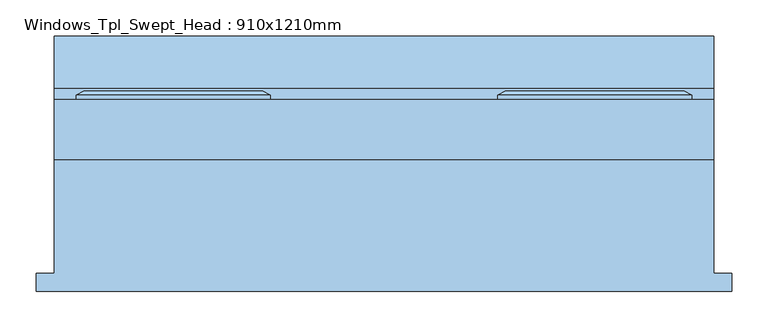
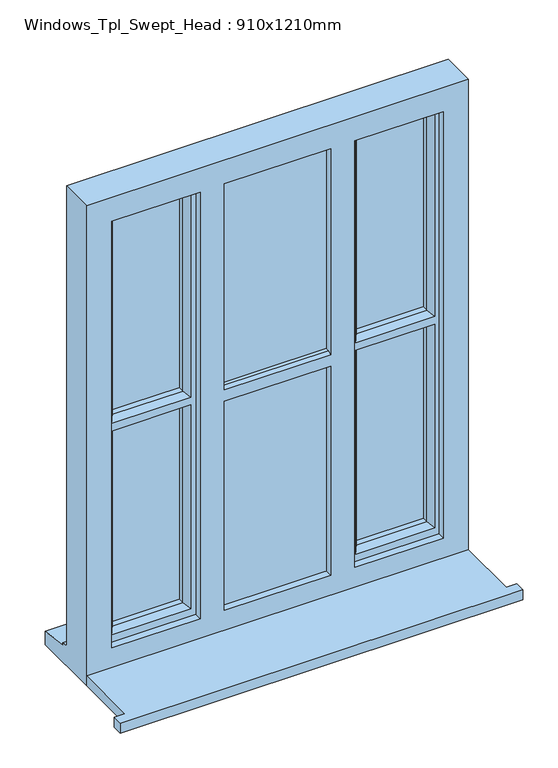
"""IFC4 building model written with IfcOpenShell, lengths in millimetres: window geometry, Windows_Tpl_Swept_Head : 910x1210mm."""

from ifc_helpers import new_model, si_unit, point, frame, frame_2d, origin, place, context, project, spatial, polyline, circle_curve, trimmed, segment, composite_curve, outline, extrude, faceted_brep, source, transform, mapped, element, save


def windows_tpl_swept_head_910x1210mm_1738034d(model_context):
    return source(origin(), model_context, "Body", "SolidModel", [
        extrude(outline(polyline([(-906.6666667, -161.5434322), (-906.6666667, -136.5434322), (-881.6666667, -136.5434322), (-881.6666667, 20.4565678), (28.3333333, 20.4565678), (28.3333333, -136.5434322), (53.3333333, -136.5434322), (53.3333333, -161.5434322), (-906.6666667, -161.5434322)])), frame((0.0, 0.0, 900.0), z_axis=(0.0, 0.0, 1.0), x_axis=(1.0, 0.0, 0.0)), (0.0, 0.0, 1.0), 25.0),
        extrude(outline(composite_curve([segment(polyline([(2050.0, -300.0), (2050.0, -553.3333333), (2013.444301, -553.3333333)]), True, "CONTINUOUS"), segment(trimmed(circle_curve(frame_2d((1325.0, -426.6666667)), 700.0), [point((2013.444301, -553.3333333))], [point((2013.444301, -300.0))], True, "CARTESIAN"), True, "CONTINUOUS"), segment(polyline([(2013.444301, -300.0), (2050.0, -300.0)]), True, "CONTINUOUS")], self_intersect=False)), frame((0.0, 62.4565678, 0.0), z_axis=(0.0, 1.0, 0.0), x_axis=(0.0, 0.0, 1.0)), (0.0, 0.0, 1.0), 25.0),
        extrude(outline(composite_curve([segment(polyline([(2030.0, -220.0), (2019.9215583, -220.0)]), True, "CONTINUOUS"), segment(trimmed(circle_curve(frame_2d((1325.0, -135.8333333)), 700.0), [point((2019.9215583, -220.0))], [point((2019.9215583, -51.6666667))], True, "CARTESIAN"), True, "CONTINUOUS"), segment(polyline([(2019.9215583, -51.6666667), (2030.0, -51.6666667), (2030.0, -220.0)]), True, "CONTINUOUS")], self_intersect=False)), frame((0.0, 79.4565678, 0.0), z_axis=(0.0, 1.0, 0.0), x_axis=(0.0, 0.0, 1.0)), (0.0, 0.0, 1.0), 24.0),
        extrude(outline(composite_curve([segment(polyline([(2030.0, -633.3333333), (2030.0, -801.6666667), (2019.9215583, -801.6666667)]), True, "CONTINUOUS"), segment(trimmed(circle_curve(frame_2d((1325.0, -717.5)), 700.0), [point((2019.9215583, -801.6666667))], [point((2019.9215583, -633.3333333))], True, "CARTESIAN"), True, "CONTINUOUS"), segment(polyline([(2019.9215583, -633.3333333), (2030.0, -633.3333333)]), True, "CONTINUOUS")], self_intersect=False)), frame((0.0, 79.4565678, 0.0), z_axis=(0.0, 1.0, 0.0), x_axis=(0.0, 0.0, 1.0)), (0.0, 0.0, 1.0), 24.0),
        faceted_brep([(-270.0, 103.4565678, 2080.0), (-270.0, 109.2300705, 2080.0), (-270.0, 109.2300705, 953.0), (-270.0, 103.4565678, 953.0), (-260.0, 38.4565678, 2070.0), (-260.0, 103.4565678, 2070.0), (-260.0, 103.4565678, 963.0), (-260.0, 38.4565678, 963.0), (-220.0, 52.9494677, 2030.0), (-230.1480377, 38.4565678, 2040.1480377), (-230.1480377, 38.4565678, 1526.3519623), (-220.0, 52.9494677, 1536.5), (-230.1480377, 38.4565678, 992.8519623), (-220.0, 52.9494677, 1003.0), (-220.0, 52.9494677, 1496.5), (-230.1480377, 38.4565678, 1506.6480377), (-220.0, 67.4565678, 2030.0), (-220.0, 67.4565678, 1536.5), (-220.0, 67.4565678, 1003.0), (-220.0, 67.4565678, 1496.5), (-230.0, 91.4565678, 1529.5), (-230.0, 91.4565678, 2040.0), (-230.0, 67.4565678, 2040.0), (-230.0, 67.4565678, 1529.5), (-230.0, 67.4565678, 1503.5), (-230.0, 67.4565678, 993.0), (-230.0, 91.4565678, 993.0), (-230.0, 91.4565678, 1503.5), (-220.0, 109.2300705, 2030.0), (-220.0, 91.4565678, 2030.0), (-220.0, 91.4565678, 1536.5), (-220.0, 109.2300705, 1536.5), (-220.0, 91.4565678, 1003.0), (-220.0, 109.2300705, 1003.0), (-220.0, 109.2300705, 1496.5), (-220.0, 91.4565678, 1496.5), (-237.4457548, 115.0035732, 2047.4457548), (-237.4457548, 115.0035732, 1519.0542452), (-237.4457548, 115.0035732, 985.5542452), (-237.4457548, 115.0035732, 1513.9457548), (-259.2153903, 115.0035732, 2069.2153903), (-259.2153903, 115.0035732, 963.7846097), (-1.6666667, 109.2300705, 953.0), (-1.6666667, 103.4565678, 953.0), (-11.6666667, 103.4565678, 963.0), (-11.6666667, 38.4565678, 963.0), (-41.5186289, 38.4565678, 992.8519623), (-51.6666667, 52.9494677, 1003.0), (-51.6666667, 67.4565678, 1003.0), (-41.6666667, 67.4565678, 993.0), (-41.6666667, 91.4565678, 993.0), (-51.6666667, 91.4565678, 1003.0), (-51.6666667, 109.2300705, 1003.0), (-34.2209119, 115.0035732, 985.5542452), (-12.4512764, 115.0035732, 963.7846097), (-1.6666667, 109.2300705, 2080.0), (-1.6666667, 103.4565678, 2080.0), (-11.6666667, 103.4565678, 2070.0), (-11.6666667, 38.4565678, 2070.0), (-41.5186289, 38.4565678, 1506.6480377), (-51.6666667, 52.9494677, 1496.5), (-41.5186289, 38.4565678, 2040.1480377), (-51.6666667, 52.9494677, 2030.0), (-51.6666667, 52.9494677, 1536.5), (-41.5186289, 38.4565678, 1526.3519623), (-51.6666667, 67.4565678, 1496.5), (-51.6666667, 67.4565678, 2030.0), (-51.6666667, 67.4565678, 1536.5), (-41.6666667, 91.4565678, 1503.5), (-41.6666667, 67.4565678, 1503.5), (-41.6666667, 67.4565678, 1529.5), (-41.6666667, 67.4565678, 2040.0), (-41.6666667, 91.4565678, 2040.0), (-41.6666667, 91.4565678, 1529.5), (-51.6666667, 91.4565678, 1496.5), (-51.6666667, 109.2300705, 1496.5), (-51.6666667, 91.4565678, 2030.0), (-51.6666667, 109.2300705, 2030.0), (-51.6666667, 109.2300705, 1536.5), (-51.6666667, 91.4565678, 1536.5), (-34.2209119, 115.0035732, 1513.9457548), (-34.2209119, 115.0035732, 2047.4457548), (-34.2209119, 115.0035732, 1519.0542452), (-12.4512764, 115.0035732, 2069.2153903)], [[[0, 1, 2, 3]], [[4, 5, 6, 7]], [[8, 9, 10, 11]], [[12, 13, 14, 15]], [[16, 8, 11, 17]], [[13, 18, 19, 14]], [[20, 21, 22, 23]], [[24, 25, 26, 27]], [[28, 29, 30, 31]], [[32, 33, 34, 35]], [[36, 28, 31, 37]], [[33, 38, 39, 34]], [[2, 1, 40, 41]], [[3, 2, 42, 43]], [[7, 6, 44, 45]], [[13, 12, 46, 47]], [[18, 13, 47, 48]], [[26, 25, 49, 50]], [[33, 32, 51, 52]], [[38, 33, 52, 53]], [[2, 41, 54, 42]], [[43, 42, 55, 56]], [[45, 44, 57, 58]], [[47, 46, 59, 60]], [[61, 62, 63, 64]], [[48, 47, 60, 65]], [[62, 66, 67, 63]], [[68, 50, 49, 69]], [[70, 71, 72, 73]], [[52, 51, 74, 75]], [[76, 77, 78, 79]], [[53, 52, 75, 80]], [[77, 81, 82, 78]], [[42, 54, 83, 55]], [[1, 0, 56, 55]], [[0, 3, 43, 56], [6, 5, 57, 44]], [[5, 4, 58, 57]], [[4, 7, 45, 58], [46, 12, 15, 59], [61, 64, 10, 9]], [[9, 8, 62, 61]], [[8, 16, 66, 62]], [[49, 25, 24, 69], [18, 48, 65, 19]], [[22, 71, 70, 23], [66, 16, 17, 67]], [[22, 21, 72, 71]], [[26, 50, 68, 27], [32, 35, 74, 51]], [[72, 21, 20, 73], [76, 79, 30, 29]], [[29, 28, 77, 76]], [[28, 36, 81, 77]], [[41, 40, 83, 54], [36, 37, 82, 81], [38, 53, 80, 39]], [[40, 1, 55, 83]], [[82, 37, 31, 78]], [[30, 79, 78, 31]], [[73, 20, 23, 70]], [[11, 63, 67, 17]], [[10, 64, 63, 11]], [[59, 15, 14, 60]], [[60, 14, 19, 65]], [[27, 68, 69, 24]], [[74, 35, 34, 75]], [[39, 80, 75, 34]]]),
        faceted_brep([(-583.3333333, 103.4565678, 2080.0), (-583.3333333, 109.2300705, 2080.0), (-851.6666667, 109.2300705, 2080.0), (-851.6666667, 103.4565678, 2080.0), (-593.3333333, 38.4565678, 2070.0), (-593.3333333, 103.4565678, 2070.0), (-841.6666667, 103.4565678, 2070.0), (-841.6666667, 38.4565678, 2070.0), (-633.3333333, 52.9494677, 2030.0), (-623.1852956, 38.4565678, 2040.1480377), (-811.8147044, 38.4565678, 2040.1480377), (-801.6666667, 52.9494677, 2030.0), (-801.6666667, 67.4565678, 2030.0), (-633.3333333, 67.4565678, 2030.0), (-623.3333333, 91.4565678, 2040.0), (-623.3333333, 67.4565678, 2040.0), (-811.6666667, 67.4565678, 2040.0), (-811.6666667, 91.4565678, 2040.0), (-633.3333333, 109.2300705, 2030.0), (-633.3333333, 91.4565678, 2030.0), (-801.6666667, 91.4565678, 2030.0), (-801.6666667, 109.2300705, 2030.0), (-819.1124215, 115.0035732, 2047.4457548), (-615.8875785, 115.0035732, 2047.4457548), (-594.117943, 115.0035732, 2069.2153903), (-840.882057, 115.0035732, 2069.2153903), (-851.6666667, 109.2300705, 953.0), (-851.6666667, 103.4565678, 953.0), (-841.6666667, 103.4565678, 963.0), (-841.6666667, 38.4565678, 963.0), (-811.8147044, 38.4565678, 1526.3519623), (-801.6666667, 52.9494677, 1536.5), (-811.8147044, 38.4565678, 992.8519623), (-801.6666667, 52.9494677, 1003.0), (-801.6666667, 52.9494677, 1496.5), (-811.8147044, 38.4565678, 1506.6480377), (-801.6666667, 67.4565678, 1536.5), (-801.6666667, 67.4565678, 1003.0), (-801.6666667, 67.4565678, 1496.5), (-811.6666667, 91.4565678, 1529.5), (-811.6666667, 67.4565678, 1529.5), (-811.6666667, 67.4565678, 1503.5), (-811.6666667, 67.4565678, 993.0), (-811.6666667, 91.4565678, 993.0), (-811.6666667, 91.4565678, 1503.5), (-801.6666667, 91.4565678, 1536.5), (-801.6666667, 109.2300705, 1536.5), (-801.6666667, 91.4565678, 1003.0), (-801.6666667, 109.2300705, 1003.0), (-801.6666667, 109.2300705, 1496.5), (-801.6666667, 91.4565678, 1496.5), (-819.1124215, 115.0035732, 1519.0542452), (-819.1124215, 115.0035732, 985.5542452), (-819.1124215, 115.0035732, 1513.9457548), (-840.882057, 115.0035732, 963.7846097), (-583.3333333, 109.2300705, 953.0), (-583.3333333, 103.4565678, 953.0), (-593.3333333, 103.4565678, 963.0), (-593.3333333, 38.4565678, 963.0), (-623.1852956, 38.4565678, 1526.3519623), (-623.1852956, 38.4565678, 1506.6480377), (-623.1852956, 38.4565678, 992.8519623), (-633.3333333, 52.9494677, 1003.0), (-633.3333333, 67.4565678, 1003.0), (-623.3333333, 67.4565678, 1529.5), (-633.3333333, 67.4565678, 1536.5), (-623.3333333, 67.4565678, 993.0), (-623.3333333, 67.4565678, 1503.5), (-633.3333333, 67.4565678, 1496.5), (-623.3333333, 91.4565678, 993.0), (-623.3333333, 91.4565678, 1529.5), (-633.3333333, 91.4565678, 1536.5), (-623.3333333, 91.4565678, 1503.5), (-633.3333333, 91.4565678, 1496.5), (-633.3333333, 91.4565678, 1003.0), (-633.3333333, 109.2300705, 1003.0), (-615.8875785, 115.0035732, 985.5542452), (-594.117943, 115.0035732, 963.7846097), (-615.8875785, 115.0035732, 1519.0542452), (-615.8875785, 115.0035732, 1513.9457548), (-633.3333333, 52.9494677, 1536.5), (-633.3333333, 52.9494677, 1496.5), (-633.3333333, 109.2300705, 1536.5), (-633.3333333, 109.2300705, 1496.5)], [[[0, 1, 2, 3]], [[4, 5, 6, 7]], [[8, 9, 10, 11]], [[8, 11, 12, 13]], [[14, 15, 16, 17]], [[18, 19, 20, 21]], [[18, 21, 22, 23]], [[2, 1, 24, 25]], [[3, 2, 26, 27]], [[7, 6, 28, 29]], [[11, 10, 30, 31]], [[32, 33, 34, 35]], [[12, 11, 31, 36]], [[33, 37, 38, 34]], [[39, 17, 16, 40]], [[41, 42, 43, 44]], [[21, 20, 45, 46]], [[47, 48, 49, 50]], [[22, 21, 46, 51]], [[48, 52, 53, 49]], [[2, 25, 54, 26]], [[27, 26, 55, 56]], [[0, 3, 27, 56], [6, 5, 57, 28]], [[29, 28, 57, 58]], [[4, 7, 29, 58], [10, 9, 59, 30], [32, 35, 60, 61]], [[33, 32, 61, 62]], [[37, 33, 62, 63]], [[16, 15, 64, 40], [13, 12, 36, 65]], [[66, 42, 41, 67], [37, 63, 68, 38]], [[43, 42, 66, 69]], [[14, 17, 39, 70], [19, 71, 45, 20]], [[43, 69, 72, 44], [47, 50, 73, 74]], [[48, 47, 74, 75]], [[52, 48, 75, 76]], [[25, 24, 77, 54], [23, 22, 51, 78], [76, 79, 53, 52]], [[26, 54, 77, 55]], [[1, 0, 56, 55]], [[5, 4, 58, 57]], [[9, 8, 80, 59]], [[62, 61, 60, 81]], [[8, 13, 65, 80]], [[63, 62, 81, 68]], [[64, 15, 14, 70]], [[72, 69, 66, 67]], [[19, 18, 82, 71]], [[75, 74, 73, 83]], [[18, 23, 78, 82]], [[76, 75, 83, 79]], [[24, 1, 55, 77]], [[78, 51, 46, 82]], [[45, 71, 82, 46]], [[40, 64, 70, 39]], [[65, 36, 31, 80]], [[30, 59, 80, 31]], [[60, 35, 34, 81]], [[38, 68, 81, 34]], [[67, 41, 44, 72]], [[73, 50, 49, 83]], [[53, 79, 83, 49]]]),
        extrude(outline(polyline([(-41.5186289, 67.4565678), (-230.0, 67.4565678), (-230.0, 91.4565678), (-41.5186289, 91.4565678), (-41.5186289, 67.4565678)])), frame((0.0, 0.0, 993.0), z_axis=(0.0, 0.0, 1.0), x_axis=(1.0, 0.0, 0.0)), (0.0, 0.0, 1.0), 513.6480377),
        extrude(outline(polyline([(-41.5186289, 67.4565678), (-230.0, 67.4565678), (-230.0, 91.4565678), (-41.5186289, 91.4565678), (-41.5186289, 67.4565678)])), frame((0.0, 0.0, 1526.3519623), z_axis=(0.0, 0.0, 1.0), x_axis=(1.0, 0.0, 0.0)), (0.0, 0.0, 1.0), 513.6480377),
        extrude(outline(polyline([(-563.3333333, 62.4565678), (-290.0, 62.4565678), (-290.0, 38.4565678), (-563.3333333, 38.4565678), (-563.3333333, 62.4565678)])), frame((0.0, 0.0, 963.0), z_axis=(0.0, 0.0, 1.0), x_axis=(1.0, 0.0, 0.0)), (0.0, 0.0, 1.0), 540.5),
        extrude(outline(polyline([(-563.3333333, 62.4565678), (-290.0, 62.4565678), (-290.0, 38.4565678), (-563.3333333, 38.4565678), (-563.3333333, 62.4565678)])), frame((0.0, 0.0, 1529.5), z_axis=(0.0, 0.0, 1.0), x_axis=(1.0, 0.0, 0.0)), (0.0, 0.0, 1.0), 540.5),
        extrude(outline(polyline([(-623.3333333, 67.4565678), (-811.6666667, 67.4565678), (-811.6666667, 91.4565678), (-623.3333333, 91.4565678), (-623.3333333, 67.4565678)])), frame((0.0, 0.0, 1526.3519623), z_axis=(0.0, 0.0, 1.0), x_axis=(1.0, 0.0, 0.0)), (0.0, 0.0, 1.0), 513.6480377),
        extrude(outline(polyline([(-623.3333333, 67.4565678), (-811.6666667, 67.4565678), (-811.6666667, 91.4565678), (-623.3333333, 91.4565678), (-623.3333333, 67.4565678)])), frame((0.0, 0.0, 993.0), z_axis=(0.0, 0.0, 1.0), x_axis=(1.0, 0.0, 0.0)), (0.0, 0.0, 1.0), 513.6480377),
        faceted_brep([(-553.3333333, 38.4565678, 2050.0), (-553.3333333, 20.4565678, 2050.0), (-553.3333333, 20.4565678, 1530.8390708), (-553.3333333, 28.5412125, 1536.5), (-553.3333333, 38.4565678, 1536.5), (-553.3333333, 20.4565678, 975.0), (-553.3333333, 38.4565678, 975.0), (-553.3333333, 38.4565678, 1496.5), (-553.3333333, 28.5412125, 1496.5), (-553.3333333, 20.4565678, 1502.1609292), (28.3333333, 20.4565678, 2110.0), (-881.6666667, 20.4565678, 2110.0), (-881.6666667, 20.4565678, 900.0), (28.3333333, 20.4565678, 900.0), (-821.6666667, 20.4565678, 2050.0), (-611.3333333, 20.4565678, 2050.0), (-611.3333333, 20.4565678, 975.0), (-821.6666667, 20.4565678, 975.0), (-242.0, 20.4565678, 2050.0), (-31.6666667, 20.4565678, 2050.0), (-31.6666667, 20.4565678, 975.0), (-242.0, 20.4565678, 975.0), (-300.0, 20.4565678, 2050.0), (-300.0, 20.4565678, 1530.8390708), (-300.0, 20.4565678, 975.0), (-300.0, 20.4565678, 1502.1609292), (-611.3333333, 38.4565678, 2050.0), (-611.3333333, 38.4565678, 975.0), (-841.6666667, 38.4565678, 2070.0), (-593.3333333, 38.4565678, 2070.0), (-593.3333333, 38.4565678, 963.0), (-841.6666667, 38.4565678, 963.0), (-821.6666667, 38.4565678, 2050.0), (-821.6666667, 38.4565678, 975.0), (-563.3333333, 38.4565678, 2070.0), (-290.0, 38.4565678, 2070.0), (-290.0, 38.4565678, 1529.5), (-553.3333333, 38.4565678, 1529.5), (-553.3333333, 38.4565678, 1503.5), (-290.0, 38.4565678, 1503.5), (-290.0, 38.4565678, 963.0), (-563.3333333, 38.4565678, 963.0), (-300.0, 38.4565678, 2050.0), (-300.0, 38.4565678, 1536.5), (-300.0, 38.4565678, 975.0), (-300.0, 38.4565678, 1496.5), (-260.0, 38.4565678, 2070.0), (-11.6666667, 38.4565678, 2070.0), (-11.6666667, 38.4565678, 963.0), (-260.0, 38.4565678, 963.0), (-31.6666667, 38.4565678, 2050.0), (-242.0, 38.4565678, 2050.0), (-242.0, 38.4565678, 975.0), (-31.6666667, 38.4565678, 975.0), (-593.3333333, 103.4565678, 2070.0), (-593.3333333, 103.4565678, 963.0), (-881.6666667, 103.4565678, 2110.0), (28.3333333, 103.4565678, 2110.0), (28.3333333, 103.4565678, 951.0), (-881.6666667, 103.4565678, 951.0), (-841.6666667, 103.4565678, 2070.0), (-841.6666667, 103.4565678, 963.0), (-553.3333333, 103.4565678, 2070.0), (-553.3333333, 103.4565678, 963.0), (-300.0, 103.4565678, 963.0), (-300.0, 103.4565678, 2070.0), (-11.6666667, 103.4565678, 963.0), (-11.6666667, 103.4565678, 2070.0), (-260.0, 103.4565678, 2070.0), (-260.0, 103.4565678, 963.0), (-553.3333333, 98.4565678, 2070.0), (-553.3333333, 98.4565678, 2050.0), (-553.3333333, 62.4565678, 2050.0), (-553.3333333, 62.4565678, 1536.5), (-553.3333333, 80.2300705, 1536.5), (-553.3333333, 86.0035732, 1519.0542452), (-553.3333333, 86.0035732, 1513.9457548), (-553.3333333, 80.2300705, 1496.5), (-553.3333333, 62.4565678, 1496.5), (-553.3333333, 62.4565678, 975.0), (-553.3333333, 98.4565678, 975.0), (-553.3333333, 98.4565678, 963.0), (-290.0, 62.4565678, 1503.5), (-553.3333333, 62.4565678, 1503.5), (-553.3333333, 62.4565678, 1529.5), (-290.0, 62.4565678, 1529.5), (-290.0, 62.4565678, 2070.0), (-563.3333333, 62.4565678, 2070.0), (-563.3333333, 62.4565678, 963.0), (-290.0, 62.4565678, 963.0), (-300.0, 62.4565678, 2050.0), (-300.0, 62.4565678, 1536.5), (-300.0, 62.4565678, 1496.5), (-300.0, 62.4565678, 975.0), (-881.6666667, 118.4565678, 949.68767), (-881.6666667, 118.4565678, 944.7449676), (-881.6666667, 190.9565678, 933.8088847), (-881.6666667, 190.9565678, 900.0), (-300.0, 98.4565678, 2070.0), (28.3333333, 190.9565678, 900.0), (28.3333333, 190.9565678, 933.8088847), (28.3333333, 118.4565678, 944.7449676), (28.3333333, 118.4565678, 949.68767), (-300.0, 98.4565678, 963.0), (-300.0, 98.4565678, 975.0), (-300.0, 80.2300705, 1496.5), (-300.0, 86.0035732, 1513.9457548), (-300.0, 86.0035732, 1519.0542452), (-300.0, 80.2300705, 1536.5), (-300.0, 98.4565678, 2050.0), (-300.0, 28.5412125, 1536.5), (-300.0, 28.5412125, 1496.5)], [[[0, 1, 2, 3, 4]], [[5, 6, 7, 8, 9]], [[10, 11, 12, 13], [14, 15, 16, 17], [18, 19, 20, 21], [1, 22, 23, 2], [24, 5, 9, 25]], [[15, 26, 27, 16]], [[28, 29, 30, 31], [26, 32, 33, 27]], [[34, 35, 36, 37, 38, 39, 40, 41], [42, 0, 4, 43], [6, 44, 45, 7]], [[46, 47, 48, 49], [50, 51, 52, 53]], [[54, 55, 30, 29]], [[56, 57, 58, 59], [55, 54, 60, 61], [62, 63, 64, 65], [66, 67, 68, 69]], [[63, 62, 70, 71, 72, 73, 74, 75, 76, 77, 78, 79, 80, 81]], [[82, 83, 84, 85, 86, 87, 88, 89], [73, 72, 90, 91], [92, 93, 79, 78]], [[88, 87, 34, 41]], [[11, 56, 59, 94, 95, 96, 97, 12]], [[61, 60, 28, 31]], [[32, 14, 17, 33]], [[11, 10, 57, 56]], [[62, 65, 98, 70]], [[87, 86, 35, 34]], [[28, 60, 54, 29]], [[67, 47, 46, 68]], [[1, 0, 42, 22]], [[14, 32, 26, 15]], [[50, 19, 18, 51]], [[57, 10, 13, 99, 100, 101, 102, 58]], [[67, 66, 48, 47]], [[19, 50, 53, 20]], [[82, 89, 40, 39]], [[35, 86, 85, 36]], [[65, 64, 103, 104, 93, 92, 105, 106, 107, 108, 91, 90, 109, 98]], [[69, 68, 46, 49]], [[51, 18, 21, 52]], [[22, 42, 43, 110, 23]], [[44, 24, 25, 111, 45]], [[99, 13, 12, 97]], [[100, 99, 97, 96]], [[101, 100, 96, 95]], [[102, 101, 95, 94]], [[58, 102, 94, 59]], [[55, 61, 31, 30]], [[64, 63, 81, 103]], [[66, 69, 49, 48]], [[89, 88, 41, 40]], [[17, 16, 27, 33]], [[21, 20, 53, 52]], [[44, 6, 5, 24]], [[83, 38, 37, 84]], [[75, 107, 106, 76]], [[76, 106, 105, 77]], [[92, 78, 77, 105]], [[38, 83, 82, 39]], [[7, 45, 111, 8]], [[25, 9, 8, 111]], [[2, 23, 110, 3]], [[43, 4, 3, 110]], [[84, 37, 36, 85]], [[73, 91, 108, 74]], [[107, 75, 74, 108]], [[79, 93, 104, 80]], [[80, 104, 103, 81]], [[109, 71, 70, 98]], [[90, 72, 71, 109]]]),
    ])


if __name__ == "__main__":
    model = new_model("IFC4")
    model_context = context("Model", 3, world=origin())
    ifc_project = project(units=[si_unit("LENGTHUNIT", "METRE", prefix="MILLI")], contexts=[model_context])
    site = spatial("IfcSite", under=ifc_project)
    building = spatial("IfcBuilding", under=site)
    placement = place(None, origin())
    windows_tpl_swept_head_910x1210mm_shape = windows_tpl_swept_head_910x1210mm_1738034d(model_context)
    element("IfcWindow", 1, ObjectType="Windows_Tpl_Swept_Head : 910x1210mm", at=placement, inside=building, context=model_context, shape_type="MappedRepresentation", body=[
        mapped(windows_tpl_swept_head_910x1210mm_shape, transform((0.0, 0.0, 0.0), x_axis=(1.0, 0.0, 0.0), y_axis=(0.0, 1.0, 0.0), z_axis=(0.0, 0.0, 1.0))),
    ])
    save(model, "model.ifc")

# Revit data of these elements
# Type "Windows_Tpl_Swept_Head : 910x1210mm"
#   Type Mark = "51"
#   Operation = "TriplePanelVertical"
#   Construction Type Id = "GSP4R"
#   Manufacturer = "Revit"
#   Keynote = "L10"
#   Analytic Construction = "1/8 in Pilkington single glazing"
#   Wrap Layers (Ext) from Ext = 102.5 mm
#   Wrap Layers (Int) from Ext = 177.5 mm
#   Window Board Projection = 25 mm
#   Window Board Extension = 25 mm
#   Visual Light Transmittance = 0.9
#   Solar Heat Gain Coefficient = 0.78
#   Rough Width = 910 mm
#   Rough Height = 1210 mm
#   Radius - Swept Head = 700 mm
#   Height = 1210 mm
#   Width = 910 mm
#   Heat Transfer Coefficient (U) = 3.6886 W/(m²·K)
#   Glazing Thickness = 24 mm
#   FrameOffset - External = 50 mm
#   Frame Depth = 65 mm
#   Default Head Height = 2110 mm
#   Cill Depth = 87.5 mm
#   Cavity Closer Width = 50 mm
#   Cavity Closer Offset from Ext = 102.5 mm
#   Cavity Closer Depth = 85 mm
#   Vis - Cavity Closers = yes
#   Material Trim = Window Frame
#   Material Glass = Glass
#   Material Frame = Window Frame
#   Wall Closure = (empty or 0)
# Element 1 (IfcWindow, "Windows_Tpl_Swept_Head : 910x1210mm")
#   Materials on its faces: "Window Frame", "Glass"
# Materials
#   "Window Frame": class "Miscellaneous", colour RGB 249 249 249, transparency 0, Keynote = "L10", Cost = 0
#   "Glass": class "Glass", colour RGB 0 128 192, transparency 0.9, Description = "Soda Lime Glass", Cost = 0
